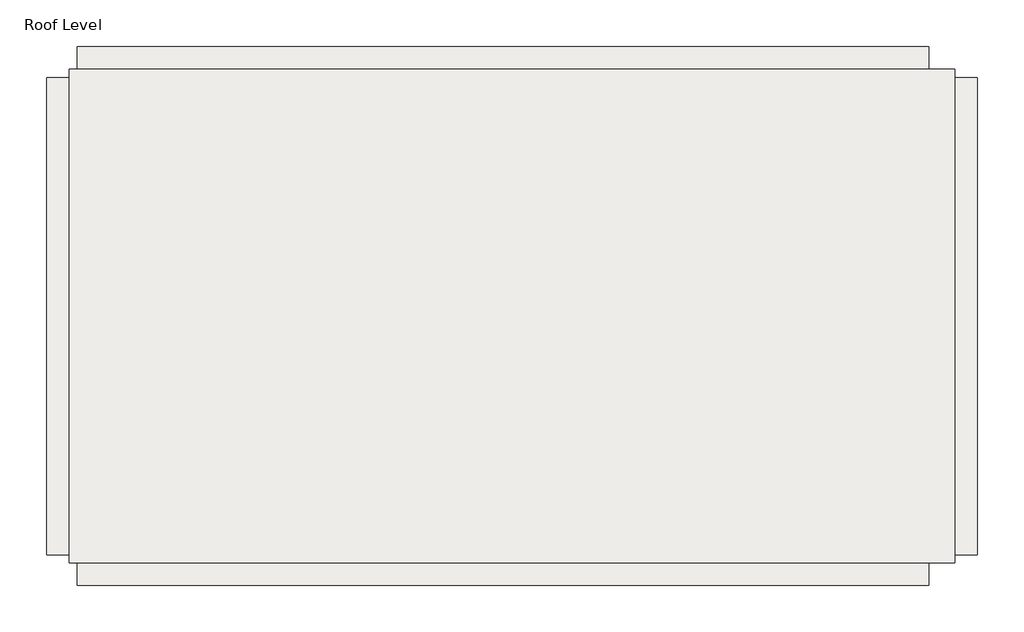
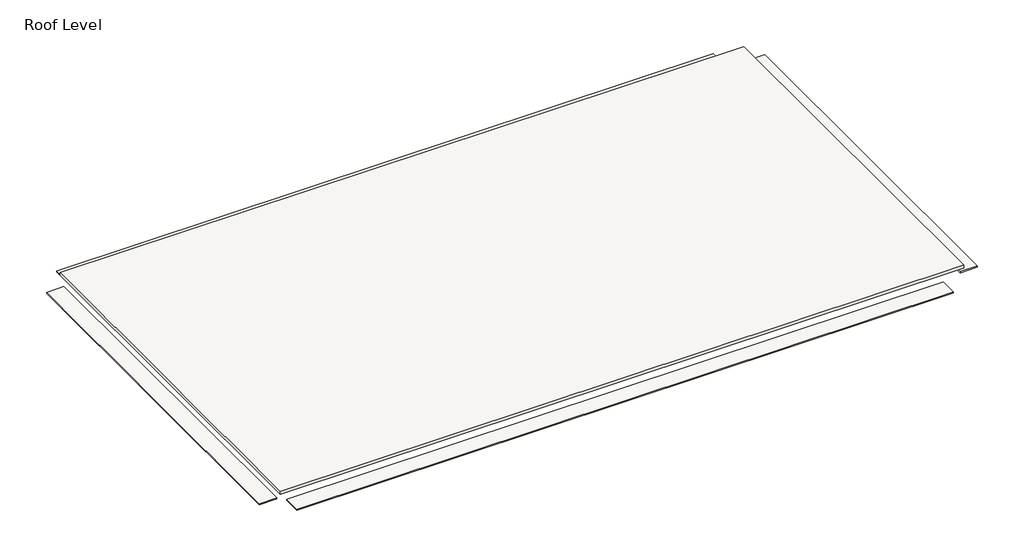
# One storey: 5 roofs.
"""IFC4 building model written with IfcOpenShell, lengths in millimetres."""

from ifc_helpers import new_model, si_unit, frame, origin, place, context, project, spatial, polyline, outline, extrude, element, save

model = new_model("IFC4")

# Units and contexts
model_context = context("Model", 3, world=origin())
ifc_project = project(units=[si_unit("LENGTHUNIT", "METRE", prefix="MILLI")], contexts=[model_context])

# Site, building, storey
site = spatial("IfcSite", under=ifc_project)
building = spatial("IfcBuilding", under=site)
storey = spatial("IfcBuildingStorey", under=building, Name="Roof Level", Elevation=7924.8)

# Roofs
placement = place(None, origin())
element("IfcRoof", 1, ObjectType="Generic - 125mm", at=placement, inside=storey, context=model_context, shape_type="SweptSolid", body=[
    extrude(outline(polyline([(1484.064681, 11296.9802217), (29068.464681, 11296.9802217), (29068.464681, -4095.4197783), (1484.064681, -4095.4197783), (1484.064681, 11296.9802217)])), frame((0.0, 0.0, 7924.8), z_axis=(0.0, 0.0, 1.0), x_axis=(1.0, 0.0, 0.0)), (0.0, 0.0, 1.0), 125.0),
])
element("IfcRoof", 2, ObjectType="Shading devices - 50mm", at=placement, inside=storey, context=model_context, shape_type="SweptSolid", body=[
    extrude(outline(polyline([(1746.464681, -4095.4197783), (28246.464681, -4095.4197783), (28246.464681, -4795.4197783), (1746.464681, -4795.4197783), (1746.464681, -4095.4197783)])), frame((0.0, 0.0, 7562.4), z_axis=(0.0, 0.0, 1.0), x_axis=(1.0, 0.0, 0.0)), (0.0, 0.0, 1.0), 50.0),
])
element("IfcRoof", 3, ObjectType="Shading devices - 50mm", at=placement, inside=storey, context=model_context, shape_type="SweptSolid", body=[
    extrude(outline(polyline([(29068.464681, 11030.5802217), (29768.464681, 11030.5802217), (29768.464681, -3843.0197783), (29068.464681, -3843.0197783), (29068.464681, 11030.5802217)])), frame((0.0, 0.0, 7562.4), z_axis=(0.0, 0.0, 1.0), x_axis=(1.0, 0.0, 0.0)), (0.0, 0.0, 1.0), 50.0),
])
element("IfcRoof", 4, ObjectType="Shading devices - 50mm", at=placement, inside=storey, context=model_context, shape_type="SweptSolid", body=[
    extrude(outline(polyline([(28246.464681, 11296.9802217), (1746.464681, 11296.9802217), (1746.464681, 11996.9802217), (28246.464681, 11996.9802217), (28246.464681, 11296.9802217)])), frame((0.0, 0.0, 7562.4), z_axis=(0.0, 0.0, 1.0), x_axis=(1.0, 0.0, 0.0)), (0.0, 0.0, 1.0), 50.0),
])
element("IfcRoof", 5, ObjectType="Shading devices - 50mm", at=placement, inside=storey, context=model_context, shape_type="SweptSolid", body=[
    extrude(outline(polyline([(784.064681, 11030.5802217), (1484.064681, 11030.5802217), (1484.064681, -3843.0197783), (784.064681, -3843.0197783), (784.064681, 11030.5802217)])), frame((0.0, 0.0, 7562.4), z_axis=(0.0, 0.0, 1.0), x_axis=(1.0, 0.0, 0.0)), (0.0, 0.0, 1.0), 50.0),
])

save(model, "model.ifc")

# Revit data of these elements
# Project information
#   Project Issue Date = "Issue Date"
#   Project Status = "Project Status"
#   Client Name = "Owner"
#   Project Address = "Enter address here"
#   Project Name = "Project Name"
#   Project Number = "Project Number"
# Type "Generic - 125mm"
#   Layers, outside or top first: 125 mm no material (function 1)
# Type "Shading devices - 50mm"
#   Layers, outside or top first: 50 mm no material (function 1)
# Element 1 (IfcRoof, "Generic - 125mm")
#   built-in parameter 1001705 = 26.4101 (stored number, unit not read)
#   built-in parameter 1001710 = 33615
#   Phase Created = New Construction
#   Materials on its faces: "Default Roof"
# Elements 2, 3, 4, 5 (IfcRoof, "Shading devices - 50mm")
#   built-in parameter 1001705 = 24.9751 (stored number, unit not read)
#   built-in parameter 1001701 = -1.18898 (stored number, unit not read)
#   built-in parameter 1001710 = 33615
#   Phase Created = New Construction
#   Materials on its faces: "Default Roof"
# Materials
#   "Default Roof": class "Miscellaneous", colour RGB 0 127 0, transparency 0, Cost = 0
